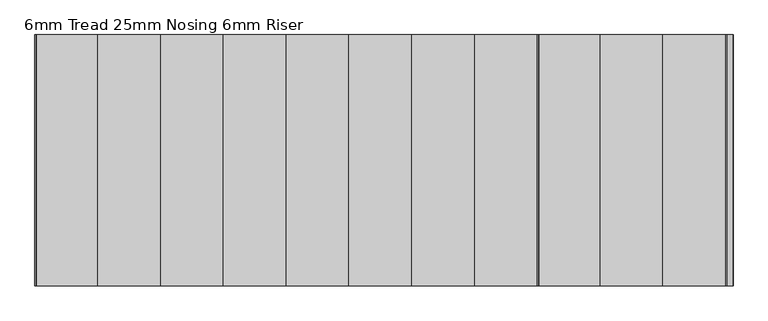
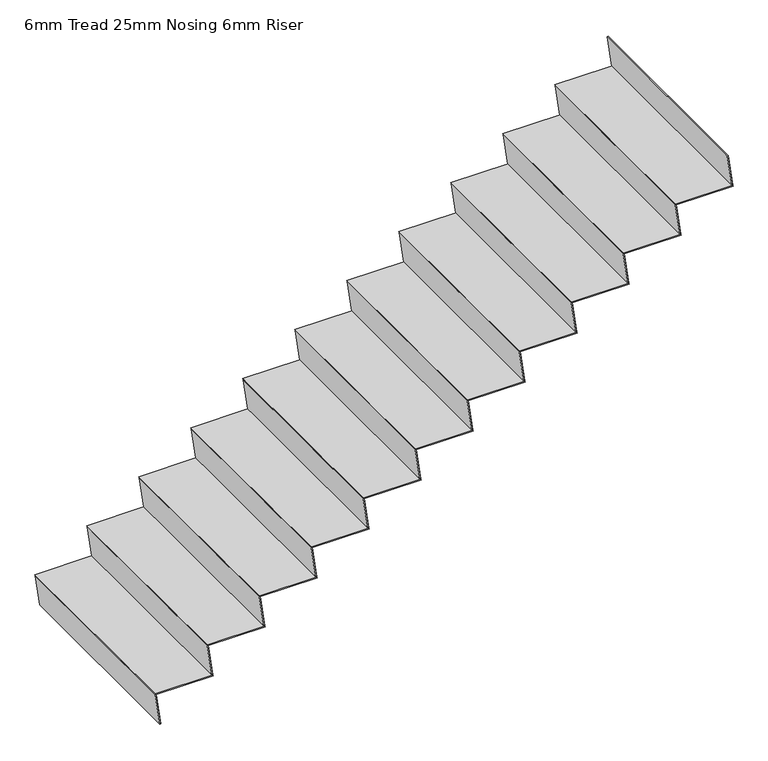
"""IFC4 building model written with IfcOpenShell, lengths in millimetres: stair flight geometry, 6mm Tread 25mm Nosing 6mm Riser."""

from ifc_helpers import new_model, si_unit, origin, place, context, project, spatial, faceted_brep, source, transform, mapped, element, save


def stair_flight_6mm_tread_25mm_nosing_6mm_riser_b4a4c334(model_context):
    return source(origin(), model_context, "Body", "Brep", [
        faceted_brep([(-16043.9409643, 12030.4345331, 2133.3333333), (-16043.0972143, 12030.4345331, 2127.3333333), (-16043.0972143, 13130.4345331, 2127.3333333), (-16043.9409643, 13130.4345331, 2133.3333333), (-16350.0, 13130.4345331, 2133.3333333), (-16350.0, 12030.4345331, 2133.3333333), (-16349.15625, 12030.4345331, 2127.3333333), (-16349.15625, 13130.4345331, 2127.3333333)], [[[0, 1, 2, 3]], [[3, 4, 5, 0]], [[2, 1, 6, 7]], [[4, 3, 2, 7]], [[0, 5, 6, 1]], [[5, 4, 7, 6]]]),
        faceted_brep([(-16349.15625, 12030.4345331, 2127.3333333), (-16325.0, 12030.4345331, 1955.5555556), (-16318.9409643, 12030.4345331, 1955.5555556), (-16343.0972143, 12030.4345331, 2127.3333333), (-16349.15625, 13130.4345331, 2127.3333333), (-16343.0972143, 13130.4345331, 2127.3333333), (-16318.9409643, 13130.4345331, 1955.5555556), (-16325.0, 13130.4345331, 1955.5555556)], [[[0, 1, 2, 3]], [[4, 5, 6, 7]], [[1, 0, 4, 7]], [[2, 1, 7, 6]], [[3, 2, 6, 5]], [[0, 3, 5, 4]]]),
        faceted_brep([(-16074.15625, 12030.4345331, 2305.1111111), (-16050.0, 12030.4345331, 2133.3333333), (-16043.9409643, 12030.4345331, 2133.3333333), (-16068.0972143, 12030.4345331, 2305.1111111), (-16074.15625, 13130.4345331, 2305.1111111), (-16068.0972143, 13130.4345331, 2305.1111111), (-16043.9409643, 13130.4345331, 2133.3333333), (-16050.0, 13130.4345331, 2133.3333333)], [[[0, 1, 2, 3]], [[4, 5, 6, 7]], [[1, 0, 4, 7]], [[2, 1, 7, 6]], [[3, 2, 6, 5]], [[0, 3, 5, 4]]]),
        faceted_brep([(-15768.9409643, 13130.4345331, 2311.1111111), (-16075.0, 13130.4345331, 2311.1111111), (-16075.0, 12030.4345331, 2311.1111111), (-15768.9409643, 12030.4345331, 2311.1111111), (-15768.0972143, 13130.4345331, 2305.1111111), (-15768.0972143, 12030.4345331, 2305.1111111), (-16074.15625, 12030.4345331, 2305.1111111), (-16074.15625, 13130.4345331, 2305.1111111)], [[[0, 1, 2, 3]], [[4, 5, 6, 7]], [[1, 0, 4, 7]], [[3, 2, 6, 5]], [[3, 5, 4, 0]], [[2, 1, 7, 6]]]),
        faceted_brep([(-15799.15625, 12030.4345331, 2482.8888889), (-15775.0, 12030.4345331, 2311.1111111), (-15768.9409643, 12030.4345331, 2311.1111111), (-15793.0972143, 12030.4345331, 2482.8888889), (-15799.15625, 13130.4345331, 2482.8888889), (-15793.0972143, 13130.4345331, 2482.8888889), (-15768.9409643, 13130.4345331, 2311.1111111), (-15775.0, 13130.4345331, 2311.1111111)], [[[0, 1, 2, 3]], [[4, 5, 6, 7]], [[1, 0, 4, 7]], [[2, 1, 7, 6]], [[3, 2, 6, 5]], [[0, 3, 5, 4]]]),
        faceted_brep([(-15493.9409643, 13130.4345331, 2488.8888889), (-15800.0, 13130.4345331, 2488.8888889), (-15800.0, 12030.4345331, 2488.8888889), (-15493.9409643, 12030.4345331, 2488.8888889), (-15493.0972143, 13130.4345331, 2482.8888889), (-15493.0972143, 12030.4345331, 2482.8888889), (-15799.15625, 12030.4345331, 2482.8888889), (-15799.15625, 13130.4345331, 2482.8888889)], [[[0, 1, 2, 3]], [[4, 5, 6, 7]], [[1, 0, 4, 7]], [[3, 2, 6, 5]], [[3, 5, 4, 0]], [[2, 1, 7, 6]]]),
        faceted_brep([(-15524.15625, 12030.4345331, 2660.6666667), (-15500.0, 12030.4345331, 2488.8888889), (-15493.9409643, 12030.4345331, 2488.8888889), (-15518.0972143, 12030.4345331, 2660.6666667), (-15524.15625, 13130.4345331, 2660.6666667), (-15518.0972143, 13130.4345331, 2660.6666667), (-15493.9409643, 13130.4345331, 2488.8888889), (-15500.0, 13130.4345331, 2488.8888889)], [[[0, 1, 2, 3]], [[4, 5, 6, 7]], [[1, 0, 4, 7]], [[2, 1, 7, 6]], [[3, 2, 6, 5]], [[0, 3, 5, 4]]]),
        faceted_brep([(-15218.9409643, 13130.4345331, 2666.6666667), (-15525.0, 13130.4345331, 2666.6666667), (-15525.0, 12030.4345331, 2666.6666667), (-15218.9409643, 12030.4345331, 2666.6666667), (-15218.0972143, 13130.4345331, 2660.6666667), (-15218.0972143, 12030.4345331, 2660.6666667), (-15524.15625, 12030.4345331, 2660.6666667), (-15524.15625, 13130.4345331, 2660.6666667)], [[[0, 1, 2, 3]], [[4, 5, 6, 7]], [[1, 0, 4, 7]], [[3, 2, 6, 5]], [[3, 5, 4, 0]], [[2, 1, 7, 6]]]),
        faceted_brep([(-15249.15625, 12030.4345331, 2838.4444444), (-15225.0, 12030.4345331, 2666.6666667), (-15218.9409643, 12030.4345331, 2666.6666667), (-15243.0972143, 12030.4345331, 2838.4444444), (-15249.15625, 13130.4345331, 2838.4444444), (-15243.0972143, 13130.4345331, 2838.4444444), (-15218.9409643, 13130.4345331, 2666.6666667), (-15225.0, 13130.4345331, 2666.6666667)], [[[0, 1, 2, 3]], [[4, 5, 6, 7]], [[1, 0, 4, 7]], [[2, 1, 7, 6]], [[3, 2, 6, 5]], [[0, 3, 5, 4]]]),
        faceted_brep([(-14943.9409643, 13130.4345331, 2844.4444444), (-15250.0, 13130.4345331, 2844.4444444), (-15250.0, 12030.4345331, 2844.4444444), (-14943.9409643, 12030.4345331, 2844.4444444), (-14943.0972143, 13130.4345331, 2838.4444444), (-14943.0972143, 12030.4345331, 2838.4444444), (-15249.15625, 12030.4345331, 2838.4444444), (-15249.15625, 13130.4345331, 2838.4444444)], [[[0, 1, 2, 3]], [[4, 5, 6, 7]], [[1, 0, 4, 7]], [[3, 2, 6, 5]], [[3, 5, 4, 0]], [[2, 1, 7, 6]]]),
        faceted_brep([(-14974.15625, 12030.4345331, 3016.2222222), (-14950.0, 12030.4345331, 2844.4444444), (-14943.9409643, 12030.4345331, 2844.4444444), (-14968.0972143, 12030.4345331, 3016.2222222), (-14974.15625, 13130.4345331, 3016.2222222), (-14968.0972143, 13130.4345331, 3016.2222222), (-14943.9409643, 13130.4345331, 2844.4444444), (-14950.0, 13130.4345331, 2844.4444444)], [[[0, 1, 2, 3]], [[4, 5, 6, 7]], [[1, 0, 4, 7]], [[2, 1, 7, 6]], [[3, 2, 6, 5]], [[0, 3, 5, 4]]]),
        faceted_brep([(-14668.9409643, 13130.4345331, 3022.2222222), (-14975.0, 13130.4345331, 3022.2222222), (-14975.0, 12030.4345331, 3022.2222222), (-14668.9409643, 12030.4345331, 3022.2222222), (-14668.0972143, 13130.4345331, 3016.2222222), (-14668.0972143, 12030.4345331, 3016.2222222), (-14974.15625, 12030.4345331, 3016.2222222), (-14974.15625, 13130.4345331, 3016.2222222)], [[[0, 1, 2, 3]], [[4, 5, 6, 7]], [[1, 0, 4, 7]], [[3, 2, 6, 5]], [[3, 5, 4, 0]], [[2, 1, 7, 6]]]),
        faceted_brep([(-14699.15625, 12030.4345331, 3194.0), (-14675.0, 12030.4345331, 3022.2222222), (-14668.9409643, 12030.4345331, 3022.2222222), (-14693.0972143, 12030.4345331, 3194.0), (-14699.15625, 13130.4345331, 3194.0), (-14693.0972143, 13130.4345331, 3194.0), (-14668.9409643, 13130.4345331, 3022.2222222), (-14675.0, 13130.4345331, 3022.2222222)], [[[0, 1, 2, 3]], [[4, 5, 6, 7]], [[1, 0, 4, 7]], [[2, 1, 7, 6]], [[3, 2, 6, 5]], [[0, 3, 5, 4]]]),
        faceted_brep([(-14393.9409643, 13130.4345331, 3200.0), (-14700.0, 13130.4345331, 3200.0), (-14700.0, 12030.4345331, 3200.0), (-14393.9409643, 12030.4345331, 3200.0), (-14393.0972143, 13130.4345331, 3194.0), (-14393.0972143, 12030.4345331, 3194.0), (-14699.15625, 12030.4345331, 3194.0), (-14699.15625, 13130.4345331, 3194.0)], [[[0, 1, 2, 3]], [[4, 5, 6, 7]], [[1, 0, 4, 7]], [[3, 2, 6, 5]], [[3, 5, 4, 0]], [[2, 1, 7, 6]]]),
        faceted_brep([(-14424.15625, 12030.4345331, 3371.7777778), (-14400.0, 12030.4345331, 3200.0), (-14393.9409643, 12030.4345331, 3200.0), (-14418.0972143, 12030.4345331, 3371.7777778), (-14424.15625, 13130.4345331, 3371.7777778), (-14418.0972143, 13130.4345331, 3371.7777778), (-14393.9409643, 13130.4345331, 3200.0), (-14400.0, 13130.4345331, 3200.0)], [[[0, 1, 2, 3]], [[4, 5, 6, 7]], [[1, 0, 4, 7]], [[2, 1, 7, 6]], [[3, 2, 6, 5]], [[0, 3, 5, 4]]]),
        faceted_brep([(-14118.9409643, 13130.4345331, 3377.7777778), (-14425.0, 13130.4345331, 3377.7777778), (-14425.0, 12030.4345331, 3377.7777778), (-14118.9409643, 12030.4345331, 3377.7777778), (-14118.0972143, 13130.4345331, 3371.7777778), (-14118.0972143, 12030.4345331, 3371.7777778), (-14424.15625, 12030.4345331, 3371.7777778), (-14424.15625, 13130.4345331, 3371.7777778)], [[[0, 1, 2, 3]], [[4, 5, 6, 7]], [[1, 0, 4, 7]], [[3, 2, 6, 5]], [[3, 5, 4, 0]], [[2, 1, 7, 6]]]),
        faceted_brep([(-14149.15625, 12030.4345331, 3549.5555556), (-14125.0, 12030.4345331, 3377.7777778), (-14118.9409643, 12030.4345331, 3377.7777778), (-14143.0972143, 12030.4345331, 3549.5555556), (-14149.15625, 13130.4345331, 3549.5555556), (-14143.0972143, 13130.4345331, 3549.5555556), (-14118.9409643, 13130.4345331, 3377.7777778), (-14125.0, 13130.4345331, 3377.7777778)], [[[0, 1, 2, 3]], [[4, 5, 6, 7]], [[1, 0, 4, 7]], [[2, 1, 7, 6]], [[3, 2, 6, 5]], [[0, 3, 5, 4]]]),
        faceted_brep([(-13843.9409643, 13130.4345331, 3555.5555556), (-14150.0, 13130.4345331, 3555.5555556), (-14150.0, 12030.4345331, 3555.5555556), (-13843.9409643, 12030.4345331, 3555.5555556), (-13843.0972143, 13130.4345331, 3549.5555556), (-13843.0972143, 12030.4345331, 3549.5555556), (-14149.15625, 12030.4345331, 3549.5555556), (-14149.15625, 13130.4345331, 3549.5555556)], [[[0, 1, 2, 3]], [[4, 5, 6, 7]], [[1, 0, 4, 7]], [[3, 2, 6, 5]], [[3, 5, 4, 0]], [[2, 1, 7, 6]]]),
        faceted_brep([(-13874.15625, 12030.4345331, 3727.3333333), (-13850.0, 12030.4345331, 3555.5555556), (-13843.9409643, 12030.4345331, 3555.5555556), (-13868.0972143, 12030.4345331, 3727.3333333), (-13874.15625, 13130.4345331, 3727.3333333), (-13868.0972143, 13130.4345331, 3727.3333333), (-13843.9409643, 13130.4345331, 3555.5555556), (-13850.0, 13130.4345331, 3555.5555556)], [[[0, 1, 2, 3]], [[4, 5, 6, 7]], [[1, 0, 4, 7]], [[2, 1, 7, 6]], [[3, 2, 6, 5]], [[0, 3, 5, 4]]]),
        faceted_brep([(-13568.9409643, 13130.4345331, 3733.3333333), (-13875.0, 13130.4345331, 3733.3333333), (-13875.0, 12030.4345331, 3733.3333333), (-13568.9409643, 12030.4345331, 3733.3333333), (-13568.0972143, 13130.4345331, 3727.3333333), (-13568.0972143, 12030.4345331, 3727.3333333), (-13874.15625, 12030.4345331, 3727.3333333), (-13874.15625, 13130.4345331, 3727.3333333)], [[[0, 1, 2, 3]], [[4, 5, 6, 7]], [[1, 0, 4, 7]], [[3, 2, 6, 5]], [[3, 5, 4, 0]], [[2, 1, 7, 6]]]),
        faceted_brep([(-13324.15625, 12030.4345331, 4082.8888889), (-13300.0, 12030.4345331, 3911.1111111), (-13293.9409643, 12030.4345331, 3911.1111111), (-13318.0972143, 12030.4345331, 4082.8888889), (-13324.15625, 13130.4345331, 4082.8888889), (-13318.0972143, 13130.4345331, 4082.8888889), (-13293.9409643, 13130.4345331, 3911.1111111), (-13300.0, 13130.4345331, 3911.1111111)], [[[0, 1, 2, 3]], [[4, 5, 6, 7]], [[1, 0, 4, 7]], [[2, 1, 7, 6]], [[3, 2, 6, 5]], [[0, 3, 5, 4]]]),
        faceted_brep([(-13599.15625, 12030.4345331, 3905.1111111), (-13575.0, 12030.4345331, 3733.3333333), (-13568.9409643, 12030.4345331, 3733.3333333), (-13593.0972143, 12030.4345331, 3905.1111111), (-13599.15625, 13130.4345331, 3905.1111111), (-13593.0972143, 13130.4345331, 3905.1111111), (-13568.9409643, 13130.4345331, 3733.3333333), (-13575.0, 13130.4345331, 3733.3333333)], [[[0, 1, 2, 3]], [[4, 5, 6, 7]], [[1, 0, 4, 7]], [[2, 1, 7, 6]], [[3, 2, 6, 5]], [[0, 3, 5, 4]]]),
        faceted_brep([(-13293.9409643, 13130.4345331, 3911.1111111), (-13325.0, 13130.4345331, 3911.1111111), (-13600.0, 13130.4345331, 3911.1111111), (-13600.0, 12030.4345331, 3911.1111111), (-13293.9409643, 12030.4345331, 3911.1111111), (-13293.0972143, 13130.4345331, 3905.1111111), (-13293.0972143, 12030.4345331, 3905.1111111), (-13599.15625, 12030.4345331, 3905.1111111), (-13599.15625, 13130.4345331, 3905.1111111), (-13325.0, 13130.4345331, 3905.1111111)], [[[0, 1, 2, 3, 4]], [[5, 6, 7, 8, 9]], [[1, 0, 5, 9]], [[2, 1, 9, 8]], [[4, 3, 7, 6]], [[4, 6, 5, 0]], [[3, 2, 8, 7]]]),
    ])


if __name__ == "__main__":
    model = new_model("IFC4")
    model_context = context("Model", 3, world=origin())
    ifc_project = project(units=[si_unit("LENGTHUNIT", "METRE", prefix="MILLI")], contexts=[model_context])
    site = spatial("IfcSite", under=ifc_project)
    building = spatial("IfcBuilding", under=site)
    placement = place(None, origin())
    stair_flight_6mm_tread_25mm_nosing_6mm_riser_shape = stair_flight_6mm_tread_25mm_nosing_6mm_riser_b4a4c334(model_context)
    element("IfcStairFlight", 1, ObjectType="6mm Tread 25mm Nosing 6mm Riser", at=placement, inside=building, context=model_context, shape_type="MappedRepresentation", body=[
        mapped(stair_flight_6mm_tread_25mm_nosing_6mm_riser_shape, transform((0.0, 0.0, 0.0), x_axis=(1.0, 0.0, 0.0), y_axis=(0.0, 1.0, 0.0), z_axis=(0.0, 0.0, 1.0))),
    ])
    save(model, "model.ifc")

# Revit data of these elements
# Element 1 (IfcStairFlight, "6mm Tread 25mm Nosing 6mm Riser")
#   Materials on its faces: "Steel, Paint Finish, Dark Gray"
# Materials
#   "Steel, Paint Finish, Dark Gray": class "Metal", colour RGB 89 89 89, transparency 0, Description = "Steel, paint finish, dark gray, glossy", Cost = 0
